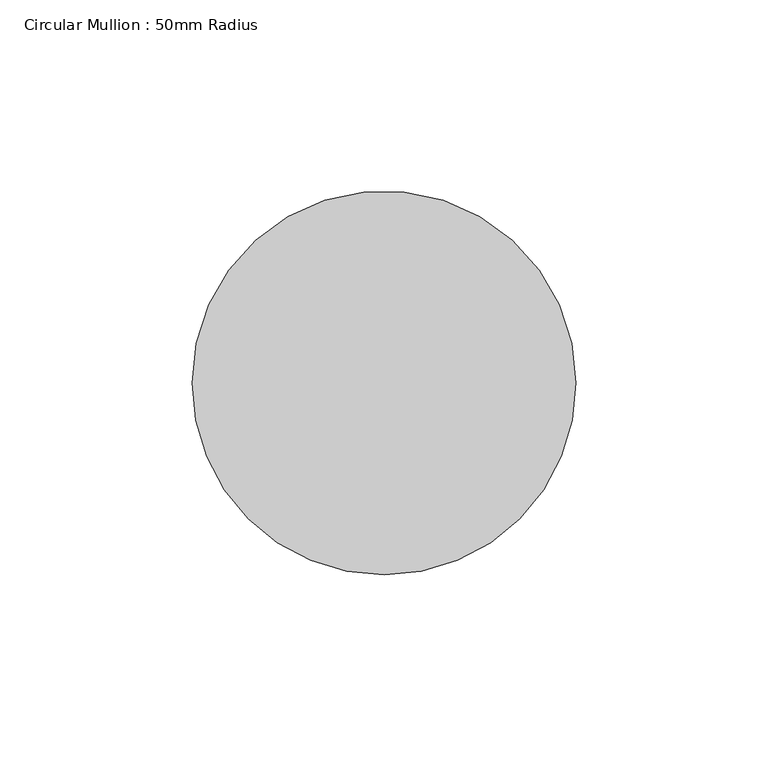
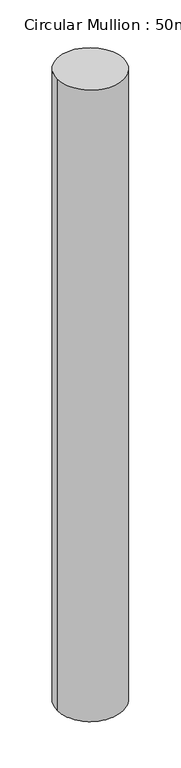
"""IFC4 building model written with IfcOpenShell, lengths in millimetres: member geometry, Circular Mullion : 50mm Radius."""

from ifc_helpers import new_model, si_unit, frame, origin, place, context, project, spatial, ellipse_curve, source, transform, mapped, element, save
from ifc_brep_helpers import plane_surface, cylinder_surface, advanced_brep


def circular_mullion_50mm_radius_d27411fe(model_context):
    return source(origin(), model_context, "Body", "AdvancedBrep", [
        advanced_brep(
        [(-100.0, 0.0, 1.7062403), (0.0, 0.0, 0.0), (0.0, 0.0, -1001.8542063), (-100.0, 0.0, -1003.5652895)],
        [
            (0, 1, ellipse_curve(frame((-50.0, 0.0, 0.8531202), z_axis=(-0.017058132266669312, -0.01447760319060743, -0.999749678234221), x_axis=(-0.7622292771307334, -0.6469203569328983, 0.022373664665657794)), 50.0125192, 50.0)),
            (1, 2),
            (2, 3, ellipse_curve(frame((-50.0, 0.0, -1002.7097479), z_axis=(-0.017106524126557807, -0.01451867440134516, 0.9997482557753903), x_axis=(0.7622281926194961, 0.6469194364849085, 0.022437136048630017)), 50.0125904, 50.0)),
            (3, 0),
            (1, 0, ellipse_curve(frame((-50.0, 0.0, 0.8531202), z_axis=(-0.017058132266669312, -0.01447760319060743, -0.999749678234221), x_axis=(-0.7622292771307334, -0.6469203569328983, 0.022373664665657794)), 50.0125192, 50.0)),
            (3, 2, ellipse_curve(frame((-50.0, 0.0, -1002.7097479), z_axis=(-0.017106524126557807, -0.01451867440134516, 0.9997482557753903), x_axis=(0.7622281926194961, 0.6469194364849085, 0.022437136048630017)), 50.0125904, 50.0)),
        ],
        [
            cylinder_surface(frame((-50.0, 0.0, 0.0), z_axis=(0.0, 0.0, 1.0), x_axis=(1.0, 0.0, 0.0)), 50.0),
            plane_surface(frame((-197.2306959, 232.3856549, 0.0), z_axis=(0.017058132266669312, 0.01447760319060743, 0.999749678234221), x_axis=(0.7622292771307334, 0.6469203569328978, -0.022373664665670468))),
            plane_surface(frame((-197.2306959, 232.3856549, -1001.8542063), z_axis=(0.01710652412655781, 0.014518674401345164, -0.9997482557753905), x_axis=(0.7622281926194961, 0.6469194364849085, 0.022437136048631068))),
        ],
        [
            (0, [[1, 2, 3, 4]]),
            (0, [[5, -4, 6, -2]]),
            (1, [[-1, -5]]),
            (2, [[-6, -3]]),
        ],
    ),
    ])


if __name__ == "__main__":
    model = new_model("IFC4")
    model_context = context("Model", 3, world=origin())
    ifc_project = project(units=[si_unit("LENGTHUNIT", "METRE", prefix="MILLI")], contexts=[model_context])
    site = spatial("IfcSite", under=ifc_project)
    building = spatial("IfcBuilding", under=site)
    placement = place(None, origin())
    circular_mullion_50mm_radius_shape = circular_mullion_50mm_radius_d27411fe(model_context)
    element("IfcMember", 1, ObjectType="Circular Mullion : 50mm Radius", at=placement, inside=building, context=model_context, shape_type="MappedRepresentation", body=[
        mapped(circular_mullion_50mm_radius_shape, transform((0.0, 0.0, 0.0), x_axis=(1.0, 0.0, 0.0), y_axis=(0.0, 1.0, 0.0), z_axis=(0.0, 0.0, 1.0))),
    ])
    save(model, "model.ifc")

# Revit data of these elements
# Type "Circular Mullion : 50mm Radius"
#   built-in parameter 1007350 = 0.164042 (stored number, unit not read)
# Element 1 (IfcMember, "Circular Mullion : 50mm Radius")
#   Materials on its faces: "Aluminium"
# Materials
#   "Aluminium": class "Metal", colour RGB 247 247 247, transparency 0, Description = "Aluminium 6061", Cost = 0
